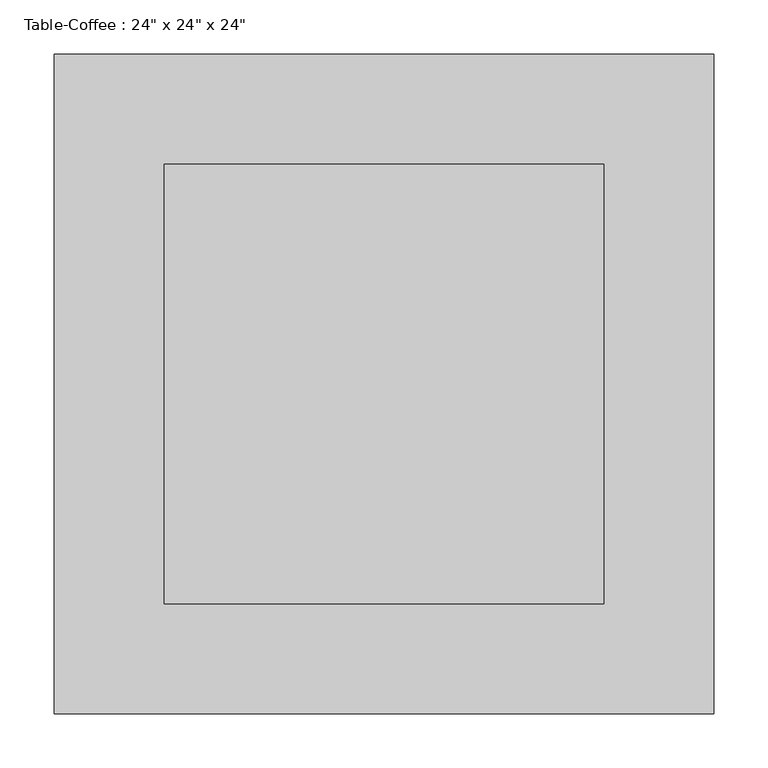
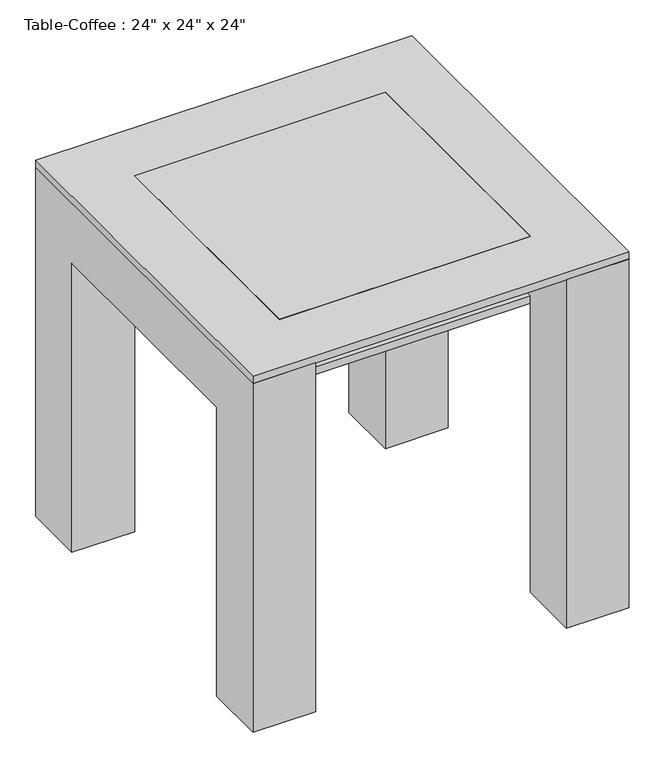
"""IFC4 building model written with IfcOpenShell, lengths in millimetres: furniture geometry."""

import ifcopenshell
import ifcopenshell.guid

model = None  # the IFC model being written
_history = None  # IfcOwnerHistory: only IFC2X3 demands one
_inside = {}  # id of a spatial element -> (the spatial element, [elements in it])
_under = {}  # id of a project, library or spatial element -> (it, [spatial elements below it])
_declared = {}  # id of a project -> (the project, [libraries it declares])
_typed = {}  # id of a type object -> (the type object, [elements of that type])
_made_of = {}  # id of a material, layer set ... -> (it, [elements and type objects made of it])


def new_model(schema):
    """Start an empty IFC model of exactly this schema.

    Asked for "IFC4X3", IfcOpenShell would pick the latest addendum, in which some entities
    have other attributes; the version numbers below select the first issue.
    IFC2X3 requires an IfcOwnerHistory on every rooted entity: one is made here for all.
    """
    global model, _history
    if schema == "IFC4X3":
        model = ifcopenshell.file(schema_version=(4, 3, 0, 0))
    else:
        model = ifcopenshell.file(schema=schema)
    _inside.clear()
    _under.clear()
    _declared.clear()
    _typed.clear()
    _made_of.clear()
    _history = None
    if model.schema == "IFC2X3":
        org = make("IfcOrganization", Name="unknown")
        user = make(
            "IfcPersonAndOrganization",
            ThePerson=make("IfcPerson", FamilyName="unknown"),
            TheOrganization=org,
        )
        app = make(
            "IfcApplication",
            ApplicationDeveloper=org,
            Version="unknown",
            ApplicationFullName="unknown",
            ApplicationIdentifier="unknown",
        )
        _history = make(
            "IfcOwnerHistory",
            OwningUser=user,
            OwningApplication=app,
            ChangeAction="ADDED",
            CreationDate=0,
        )
    return model


def make(cls, **values):
    """One entity of the class cls with the attributes given. An attribute that is None is left unset."""
    return model.create_entity(
        cls, **{name: value for name, value in values.items() if value is not None}
    )


def rooted(cls, **values):
    """An entity with a GlobalId (a new one), such as an element, a storey or a relation."""
    return make(cls, GlobalId=ifcopenshell.guid.new(), OwnerHistory=_history, **values)


def si_unit(unit_type, name, prefix=None):
    """IfcSIUnit, for example si_unit("LENGTHUNIT", "METRE", prefix="MILLI")."""
    return make("IfcSIUnit", UnitType=unit_type, Prefix=prefix, Name=name)


def assignment(units):
    """IfcUnitAssignment: the units of a project."""
    return None if units is None else make("IfcUnitAssignment", Units=units)


def point(xyz):
    """IfcCartesianPoint."""
    return None if xyz is None else make("IfcCartesianPoint", Coordinates=xyz)


def direction(xyz):
    """IfcDirection."""
    return None if xyz is None else make("IfcDirection", DirectionRatios=xyz)


def frame(location, z_axis=None, x_axis=None):
    """IfcAxis2Placement3D, a coordinate frame: its origin and axes. An axis left out is left unset."""
    return make(
        "IfcAxis2Placement3D",
        Location=point(location),
        Axis=direction(z_axis),
        RefDirection=direction(x_axis),
    )


def origin():
    """The frame at (0, 0, 0) with its axes left unset."""
    return frame((0.0, 0.0, 0.0))


def place(relative_to, where):
    """IfcLocalPlacement: puts the frame where relative to a parent placement (None: the world)."""
    return make(
        "IfcLocalPlacement", PlacementRelTo=relative_to, RelativePlacement=where
    )


def context(
    kind, dimensions, precision=None, world=None, true_north=None, identifier=None
):
    """IfcGeometricRepresentationContext, for example the 3D "Model" context."""
    return make(
        "IfcGeometricRepresentationContext",
        ContextIdentifier=identifier,
        ContextType=kind,
        CoordinateSpaceDimension=dimensions,
        Precision=precision,
        WorldCoordinateSystem=world,
        TrueNorth=true_north,
    )


def project(units=None, contexts=None):
    """IfcProject with its units and contexts."""
    return rooted(
        "IfcProject",
        Name="project",
        RepresentationContexts=contexts,
        UnitsInContext=assignment(units),
    )


def spatial(cls, under=None, at=None, **own):
    """A site, building, storey or space (cls), placed at a placement, below another one or the project."""
    s = rooted(cls, ObjectPlacement=at, **own)
    if under is not None:
        _under.setdefault(under.id(), (under, []))[1].append(s)
    return s


def polyline(points):
    """IfcPolyline through the points."""
    return make("IfcPolyline", Points=[point(p) for p in points])


def outline(outer, holes=None, kind="AREA"):
    """IfcArbitraryClosedProfileDef: a profile drawn as a closed curve; with holes, ...WithVoids."""
    if holes is None:
        return make("IfcArbitraryClosedProfileDef", ProfileType=kind, OuterCurve=outer)
    return make(
        "IfcArbitraryProfileDefWithVoids",
        ProfileType=kind,
        OuterCurve=outer,
        InnerCurves=holes,
    )


def extrude(swept, where, along, depth):
    """IfcExtrudedAreaSolid: the profile swept, set in the frame where, extruded along a direction by depth."""
    return make(
        "IfcExtrudedAreaSolid",
        SweptArea=swept,
        Position=where,
        ExtrudedDirection=direction(along),
        Depth=depth,
    )


def shape(context_of_items, identifier, shape_type, items):
    """IfcShapeRepresentation: the items that make up one representation, for example the "Body"."""
    return make(
        "IfcShapeRepresentation",
        ContextOfItems=context_of_items,
        RepresentationIdentifier=identifier,
        RepresentationType=shape_type,
        Items=items,
    )


def source(mapping_origin, context_of_items, identifier, shape_type, items):
    """IfcRepresentationMap: a shape defined once, which mapped items show again and again."""
    return make(
        "IfcRepresentationMap",
        MappingOrigin=mapping_origin,
        MappedRepresentation=shape(context_of_items, identifier, shape_type, items),
    )


def transform(
    local_origin,
    x_axis=None,
    y_axis=None,
    z_axis=None,
    scale=None,
    scale2=None,
    scale3=None,
    uniform=True,
):
    """IfcCartesianTransformationOperator3D, or its non-uniform kind. x_axis, y_axis, z_axis: its Axis1, 2, 3."""
    if uniform:
        return make(
            "IfcCartesianTransformationOperator3D",
            Axis1=direction(x_axis),
            Axis2=direction(y_axis),
            LocalOrigin=point(local_origin),
            Scale=scale,
            Axis3=direction(z_axis),
        )
    return make(
        "IfcCartesianTransformationOperator3DnonUniform",
        Axis1=direction(x_axis),
        Axis2=direction(y_axis),
        LocalOrigin=point(local_origin),
        Scale=scale,
        Axis3=direction(z_axis),
        Scale2=scale2,
        Scale3=scale3,
    )


def mapped(mapping_source, mapping_target):
    """IfcMappedItem: shows the shape of a source again, moved by a transform."""
    return make(
        "IfcMappedItem", MappingSource=mapping_source, MappingTarget=mapping_target
    )


def made_of(thing, what):
    """Note that an element or type object is made of a material, layer set ...; save() writes the relation."""
    if what is not None:
        _made_of.setdefault(what.id(), (what, []))[1].append(thing)
    return thing


def element(
    cls,
    number,
    at=None,
    inside=None,
    cuts=None,
    type_object=None,
    material=None,
    context=None,
    identifier="Body",
    shape_type=None,
    held_by="IfcProductDefinitionShape",
    body=None,
    shapes=None,
    **own,
):
    """One element of the class cls, such as IfcWall. Its Tag is "e" and its number.

    at: its placement. inside: the storey or other place that contains it. cuts: it is an
    opening in that element (IfcRelVoidsElement). A single representation is given by context,
    identifier, shape_type and body (its items); several are given by shapes. held_by: the class
    of the entity that holds the representations. save() writes the other relations.
    """
    e = rooted(cls, Tag="e%d" % number, ObjectPlacement=at, **own)
    if body is not None:
        shapes = [shape(context, identifier, shape_type, body)]
    if shapes is not None:
        e.Representation = make(held_by, Representations=shapes)
    if inside is not None:
        _inside.setdefault(inside.id(), (inside, []))[1].append(e)
    if cuts is not None:
        rooted(
            "IfcRelVoidsElement", RelatingBuildingElement=cuts, RelatedOpeningElement=e
        )
    if type_object is not None:
        _typed.setdefault(type_object.id(), (type_object, []))[1].append(e)
    return made_of(e, material)


def aggregate(whole, parts):
    """IfcRelAggregates: a whole, such as a stair, and the parts it consists of."""
    return rooted("IfcRelAggregates", RelatingObject=whole, RelatedObjects=parts)


def save(model, path):
    """Write the relations noted so far, then the file.

    IfcRelAggregates (storeys below a building ...), IfcRelContainedInSpatialStructure (elements
    in a storey), IfcRelDefinesByType, IfcRelAssociatesMaterial and IfcRelDeclares: one each for
    every whole, place, type object, material and project.
    """
    for whole, parts in _under.values():
        aggregate(whole, parts)
    for where, things in _inside.values():
        rooted(
            "IfcRelContainedInSpatialStructure",
            RelatedElements=things,
            RelatingStructure=where,
        )
    for kind, things in _typed.values():
        rooted("IfcRelDefinesByType", RelatedObjects=things, RelatingType=kind)
    for what, things in _made_of.values():
        rooted("IfcRelAssociatesMaterial", RelatedObjects=things, RelatingMaterial=what)
    for by, libraries in _declared.values():
        rooted("IfcRelDeclares", RelatingContext=by, RelatedDefinitions=libraries)
    model.write(path)


def furniture_b5c51a22(model_context):
    return source(origin(), model_context, "Body", "SweptSolid", [
        extrude(outline(polyline([(221.4657667, 298.4110778), (221.4657667, -107.9889222), (-184.9342333, -107.9889222), (-184.9342333, 298.4110778), (221.4657667, 298.4110778)])), frame((0.0, 0.0, 495.3), z_axis=(0.0, 0.0, 1.0), x_axis=(1.0, 0.0, 0.0)), (0.0, 0.0, 1.0), 12.7),
        extrude(outline(polyline([(400.0110778, 0.0), (298.4110778, 0.0), (298.4110778, 495.3), (-107.9889222, 495.3), (-107.9889222, 0.0), (-209.5889222, 0.0), (-209.5889222, 596.9), (400.0110778, 596.9), (400.0110778, 0.0)])), frame((221.4657667, 0.0, 0.0), z_axis=(1.0, 0.0, 0.0), x_axis=(0.0, 1.0, 0.0)), (0.0, 0.0, 1.0), 101.6),
        extrude(outline(polyline([(400.0110778, 596.9), (400.0110778, 0.0), (298.4110778, 0.0), (298.4110778, 495.3), (-107.9889222, 495.3), (-107.9889222, 0.0), (-209.5889222, 0.0), (-209.5889222, 596.9), (400.0110778, 596.9)])), frame((-286.5342333, 0.0, 0.0), z_axis=(1.0, 0.0, 0.0), x_axis=(0.0, 1.0, 0.0)), (0.0, 0.0, 1.0), 101.6),
        extrude(outline(polyline([(221.4657667, 298.4110778), (221.4657667, -107.9889222), (-184.9342333, -107.9889222), (-184.9342333, 298.4110778), (221.4657667, 298.4110778)])), frame((0.0, 0.0, 596.9), z_axis=(0.0, 0.0, 1.0), x_axis=(1.0, 0.0, 0.0)), (0.0, 0.0, 1.0), 12.7),
        extrude(outline(polyline([(323.0657667, 400.0110778), (323.0657667, -209.5889222), (-286.5342333, -209.5889222), (-286.5342333, 400.0110778), (323.0657667, 400.0110778)]), holes=[polyline([(221.4657667, 298.4110778), (-184.9342333, 298.4110778), (-184.9342333, -107.9889222), (221.4657667, -107.9889222), (221.4657667, 298.4110778)])]), frame((0.0, 0.0, 596.9), z_axis=(0.0, 0.0, 1.0), x_axis=(1.0, 0.0, 0.0)), (0.0, 0.0, 1.0), 12.7),
    ])


if __name__ == "__main__":
    model = new_model("IFC4")
    model_context = context("Model", 3, world=origin())
    ifc_project = project(units=[si_unit("LENGTHUNIT", "METRE", prefix="MILLI")], contexts=[model_context])
    site = spatial("IfcSite", under=ifc_project)
    building = spatial("IfcBuilding", under=site)
    placement = place(None, origin())
    furniture_shape = furniture_b5c51a22(model_context)
    element("IfcFurniture", 1, ObjectType="Table-Coffee : 24\" x 24\" x 24\"", at=placement, inside=building, context=model_context, shape_type="MappedRepresentation", body=[
        mapped(furniture_shape, transform((0.0, 0.0, 0.0), x_axis=(1.0, 0.0, 0.0), y_axis=(0.0, 1.0, 0.0), z_axis=(0.0, 0.0, 1.0))),
    ])
    save(model, "model.ifc")

# Revit data of these elements
# Type "Table-Coffee : 24\" x 24\" x 24\""
#   Model = "TBL-2424"
#   Manufacturer = "Acme Furniture"
#   Type Mark = "TB-3"
#   Assembly Code = "E2020200"
#   Cost = 1250
#   Height = 2' - 0"
#   Length = 2' - 0"
#   Width = 2' - 0"
#   Top Material = none
#   Frame Material = none
#   Default Elevation = 0
# Element 1 (IfcFurniture, "Table-Coffee : 24\" x 24\" x 24\"")
#   Materials on its faces: "Glass - Clear, Grey"
# Materials
#   "Glass - Clear, Grey": class "Glass", colour RGB 252 255 255, transparency 0.64
